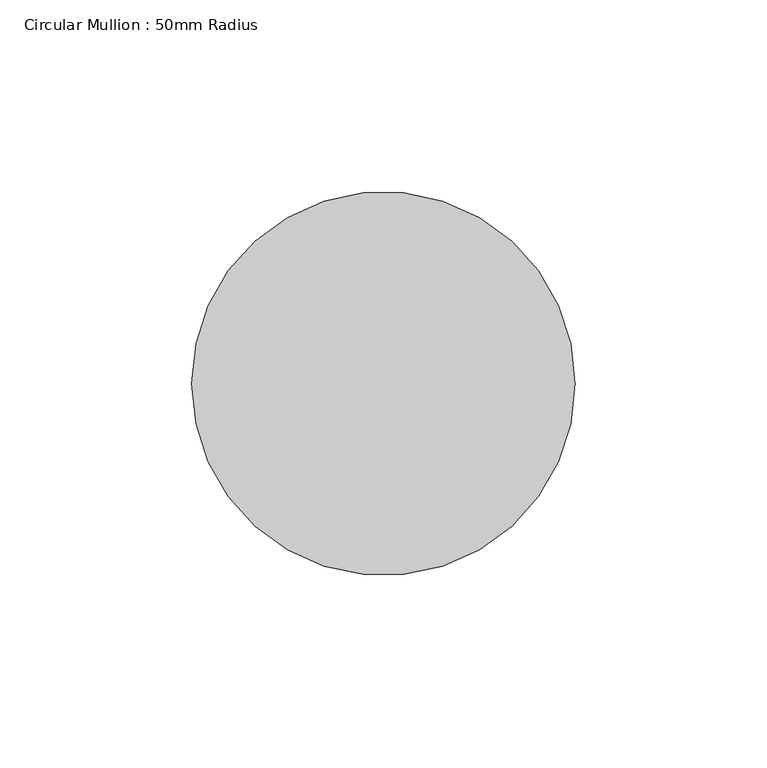
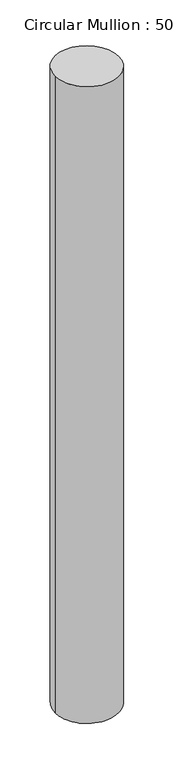
"""IFC4 building model written with IfcOpenShell, lengths in millimetres: member geometry, Circular Mullion : 50mm Radius."""

from ifc_helpers import new_model, si_unit, frame, origin, place, context, project, spatial, ellipse_curve, source, transform, mapped, element, save
from ifc_brep_helpers import plane_surface, cylinder_surface, advanced_brep


def circular_mullion_50mm_radius_14ec3c07(model_context):
    return source(origin(), model_context, "Body", "AdvancedBrep", [
        advanced_brep(
        [(-100.0, 0.0, 1.3209986), (0.0, 0.0, 0.0), (0.0, 0.0, -1052.9435835), (-100.0, 0.0, -1054.2259065)],
        [
            (0, 1, ellipse_curve(frame((-50.0, 0.0, 0.6604993), z_axis=(-0.013207354734198505, -0.014964567815430678, -0.9998007939039768), x_axis=(-0.661583460678459, -0.7496058644699468, 0.019959271253674762)), 50.0099623, 50.0)),
            (1, 2),
            (2, 3, ellipse_curve(frame((-50.0, 0.0, -1053.584745), z_axis=(-0.01282082339269373, -0.014526609224240528, 0.9998122844374235), x_axis=(0.6615910641399987, 0.7496144795573814, 0.019375135819409094)), 50.0093875, 50.0)),
            (3, 0),
            (1, 0, ellipse_curve(frame((-50.0, 0.0, 0.6604993), z_axis=(-0.013207354734198505, -0.014964567815430678, -0.9998007939039768), x_axis=(-0.661583460678459, -0.7496058644699468, 0.019959271253674762)), 50.0099623, 50.0)),
            (3, 2, ellipse_curve(frame((-50.0, 0.0, -1053.584745), z_axis=(-0.01282082339269373, -0.014526609224240528, 0.9998122844374235), x_axis=(0.6615910641399987, 0.7496144795573814, 0.019375135819409094)), 50.0093875, 50.0)),
        ],
        [
            cylinder_surface(frame((-50.0, 0.0, 0.0), z_axis=(0.0, 0.0, 1.0), x_axis=(1.0, 0.0, 0.0)), 50.0),
            plane_surface(frame((-228.5253911, 201.6908169, 0.0), z_axis=(0.013207354734198509, 0.014964567815430681, 0.999800793903977), x_axis=(0.661583460678459, 0.7496058644699469, -0.019959271253670047))),
            plane_surface(frame((-228.5253911, 201.6908169, -1052.9435835), z_axis=(0.012820823392693734, 0.014526609224240532, -0.9998122844374238), x_axis=(0.6615910641399987, 0.7496144795573815, 0.01937513581940609))),
        ],
        [
            (0, [[1, 2, 3, 4]]),
            (0, [[5, -4, 6, -2]]),
            (1, [[-1, -5]]),
            (2, [[-6, -3]]),
        ],
    ),
    ])


if __name__ == "__main__":
    model = new_model("IFC4")
    model_context = context("Model", 3, world=origin())
    ifc_project = project(units=[si_unit("LENGTHUNIT", "METRE", prefix="MILLI")], contexts=[model_context])
    site = spatial("IfcSite", under=ifc_project)
    building = spatial("IfcBuilding", under=site)
    placement = place(None, origin())
    circular_mullion_50mm_radius_shape = circular_mullion_50mm_radius_14ec3c07(model_context)
    element("IfcMember", 1, ObjectType="Circular Mullion : 50mm Radius", at=placement, inside=building, context=model_context, shape_type="MappedRepresentation", body=[
        mapped(circular_mullion_50mm_radius_shape, transform((0.0, 0.0, 0.0), x_axis=(1.0, 0.0, 0.0), y_axis=(0.0, 1.0, 0.0), z_axis=(0.0, 0.0, 1.0))),
    ])
    save(model, "model.ifc")

# Revit data of these elements
# Type "Circular Mullion : 50mm Radius"
#   built-in parameter 1007350 = 0.164042 (stored number, unit not read)
# Element 1 (IfcMember, "Circular Mullion : 50mm Radius")
#   Materials on its faces: "Aluminium"
# Materials
#   "Aluminium": class "Metal", colour RGB 247 247 247, transparency 0, Description = "Aluminium 6061", Cost = 0
